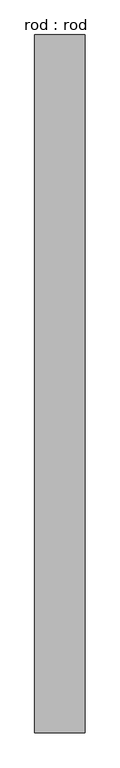
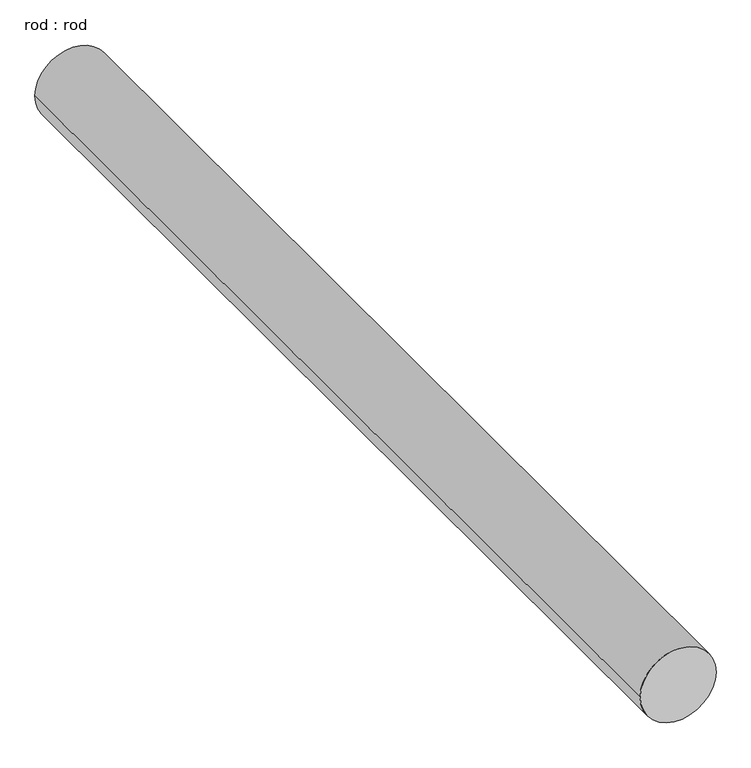
"""IFC4 building model written with IfcOpenShell, lengths in millimetres: proxy geometry, rod : rod."""

from ifc_helpers import new_model, si_unit, point, frame, frame_2d, origin, place, context, project, spatial, circle_curve, trimmed, segment, composite_curve, outline, extrude, source, transform, mapped, element, save


def rod_rod_c99de74c(model_context):
    return source(origin(), model_context, "Body", "SweptSolid", [
        extrude(outline(composite_curve([segment(trimmed(circle_curve(frame_2d((0.0108462, 0.0)), 200.0), [point((0.0108462, 200.0))], [point((0.0108462, -200.0))], False, "CARTESIAN"), True, "CONTINUOUS"), segment(trimmed(circle_curve(frame_2d((0.0108462, 0.0)), 200.0), [point((0.0108462, -200.0))], [point((0.0108462, 200.0))], False, "CARTESIAN"), True, "CONTINUOUS")], self_intersect=False)), frame((0.0, 1328.9212324, 0.0), z_axis=(0.0, 1.0, 0.0), x_axis=(0.0, 0.0, 1.0)), (0.0, 0.0, 1.0), 5527.6147659),
    ])


if __name__ == "__main__":
    model = new_model("IFC4")
    model_context = context("Model", 3, world=origin())
    ifc_project = project(units=[si_unit("LENGTHUNIT", "METRE", prefix="MILLI")], contexts=[model_context])
    site = spatial("IfcSite", under=ifc_project)
    building = spatial("IfcBuilding", under=site)
    placement = place(None, origin())
    rod_rod_shape = rod_rod_c99de74c(model_context)
    element("IfcBuildingElementProxy", 1, Name="rod : rod", ObjectType="rod : rod", at=placement, inside=building, context=model_context, shape_type="MappedRepresentation", body=[
        mapped(rod_rod_shape, transform((0.0, 0.0, 0.0), x_axis=(1.0, 0.0, 0.0), y_axis=(0.0, 1.0, 0.0), z_axis=(0.0, 0.0, 1.0))),
    ])
    save(model, "model.ifc")

# Revit data of these elements
# Type "rod : rod"
#   Default Elevation = 0
